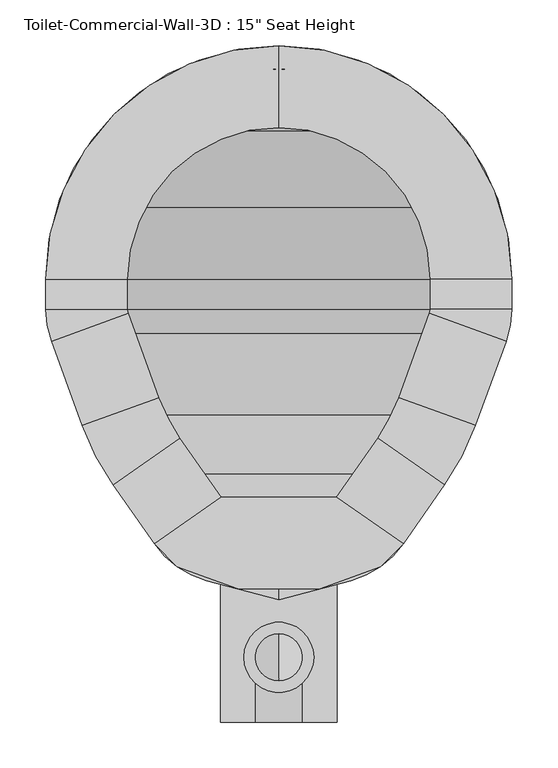
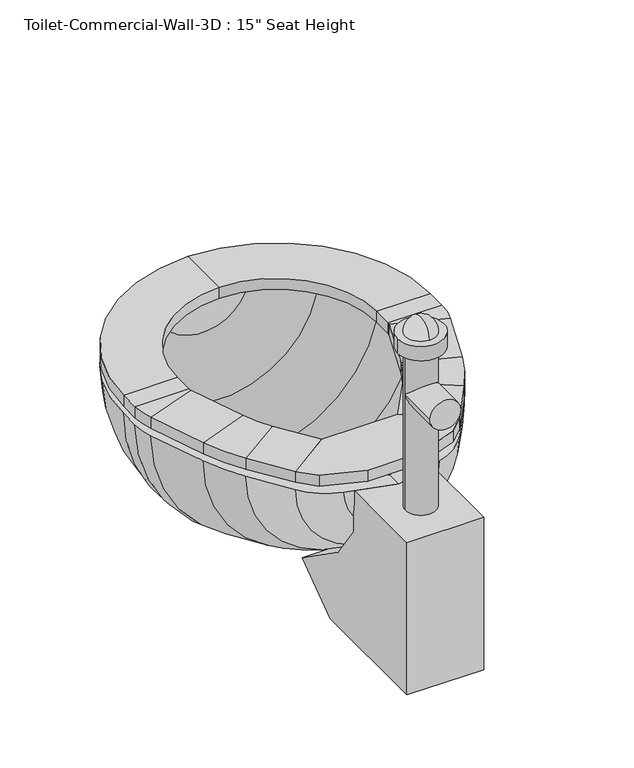
"""IFC4 building model written with IfcOpenShell, lengths in millimetres: flow terminal geometry."""

from ifc_helpers import new_model, si_unit, point, frame, frame_2d, origin, place, context, project, spatial, polyline, circle_curve, ellipse_curve, trimmed, segment, composite_curve, outline, extrude, source, transform, mapped, element, save
from ifc_brep_helpers import plane_surface, cylinder_surface, revolved_surface, advanced_brep


def flow_terminal_fb6ce90a(model_context):
    return source(origin(), model_context, "Body", "SolidModel", [
        extrude(outline(polyline([(467.7541169, 443.4722495), (540.5767337, 392.4813043), (515.6262519, 367.5308226), (449.563909, 343.4860961), (360.2423986, 343.4860961), (294.1800557, 367.5308226), (269.229574, 392.4813043), (342.0521907, 443.4722495), (467.7541169, 443.4722495)])), frame((0.0, 0.0, 355.6), z_axis=(0.0, 0.0, 1.0), x_axis=(1.0, 0.0, 0.0)), (0.0, 0.0, 1.0), 19.05),
        advanced_brep(
        [(467.7541169, 443.4722495, 355.6), (540.5767337, 392.4813043, 355.6), (540.5767337, 392.4813043, 374.65), (467.7541169, 443.4722495, 374.65), (512.8583992, 507.8878403, 355.6), (585.6810159, 456.8968951, 355.6), (585.6810159, 456.8968951, 374.65), (512.8583992, 507.8878403, 374.65), (619.360053, 521.5937234, 355.6), (535.821379, 551.9993141, 355.6), (619.360053, 521.5937234, 374.65), (535.821379, 551.9993141, 374.65), (569.2372501, 643.8086654, 355.6), (652.7759241, 613.4030747, 355.6), (652.7759241, 613.4030747, 374.65), (569.2372501, 643.8086654, 374.65), (658.9031538, 648.1523212, 355.6), (570.0031538, 648.1523212, 355.6), (658.9031538, 648.1523212, 374.65), (570.0031538, 648.1523212, 374.65), (570.0031538, 681.0375, 355.6), (658.9031538, 681.0375, 355.6), (658.9031538, 681.0375, 374.65), (570.0031538, 681.0375, 374.65), (404.9031538, 935.0375, 355.6), (404.9031538, 846.1375, 355.6), (404.9031538, 935.0375, 374.65), (404.9031538, 846.1375, 374.65), (150.9031538, 681.0375, 355.6), (239.8031538, 681.0375, 355.6), (150.9031538, 681.0375, 374.65), (239.8031538, 681.0375, 374.65), (239.8031538, 648.1523212, 355.6), (150.9031538, 648.1523212, 355.6), (150.9031538, 648.1523212, 374.65), (239.8031538, 648.1523212, 374.65), (157.0303835, 613.4030747, 355.6), (240.5690575, 643.8086654, 355.6), (157.0303835, 613.4030747, 374.65), (240.5690575, 643.8086654, 374.65), (273.9849286, 551.9993141, 355.6), (190.4462546, 521.5937234, 355.6), (190.4462546, 521.5937234, 374.65), (273.9849286, 551.9993141, 374.65), (224.1252917, 456.8968951, 355.6), (296.9479084, 507.8878403, 355.6), (224.1252917, 456.8968951, 374.65), (296.9479084, 507.8878403, 374.65), (342.0521907, 443.4722495, 355.6), (342.0521907, 443.4722495, 374.65), (269.229574, 392.4813043, 374.65), (269.229574, 392.4813043, 355.6)],
        [
            (0, 1),
            (1, 2),
            (2, 3),
            (3, 0),
            (0, 4),
            (4, 5),
            (5, 1),
            (5, 6),
            (6, 2),
            (6, 7),
            (7, 3),
            (7, 4),
            (8, 5, circle_curve(frame((356.8099347, 617.1541514, 355.6), z_axis=(0.0, 0.0, -1.0), x_axis=(0.81915204428899, -0.5735764363510486, 0.0)), 279.4)),
            (4, 9, circle_curve(frame((356.8099347, 617.1541514, 355.6), z_axis=(0.0, 0.0, 1.0), x_axis=(0.81915204428899, -0.5735764363510486, 0.0)), 190.5)),
            (9, 8),
            (10, 6, circle_curve(frame((356.8099347, 617.1541514, 374.65), z_axis=(0.0, 0.0, -1.0), x_axis=(0.81915204428899, -0.5735764363510486, 0.0)), 279.4)),
            (8, 10),
            (11, 7, circle_curve(frame((356.8099347, 617.1541514, 374.65), z_axis=(0.0, 0.0, -1.0), x_axis=(0.81915204428899, -0.5735764363510486, 0.0)), 190.5)),
            (10, 11),
            (11, 9),
            (9, 12),
            (12, 13),
            (13, 8),
            (13, 14),
            (14, 10),
            (14, 15),
            (15, 11),
            (15, 12),
            (16, 13, circle_curve(frame((557.3031538, 648.1523212, 355.6), z_axis=(0.0, 0.0, -1.0), x_axis=(0.9396926207859057, -0.3420201433256761, 0.0)), 101.6)),
            (12, 17, circle_curve(frame((557.3031538, 648.1523212, 355.6), z_axis=(0.0, 0.0, 1.0), x_axis=(0.9396926207859057, -0.3420201433256761, 0.0)), 12.7)),
            (17, 16),
            (18, 14, circle_curve(frame((557.3031538, 648.1523212, 374.65), z_axis=(0.0, 0.0, -1.0), x_axis=(0.9396926207859057, -0.3420201433256761, 0.0)), 101.6)),
            (16, 18),
            (19, 15, circle_curve(frame((557.3031538, 648.1523212, 374.65), z_axis=(0.0, 0.0, -1.0), x_axis=(0.9396926207859057, -0.3420201433256761, 0.0)), 12.7)),
            (18, 19),
            (19, 17),
            (17, 20),
            (20, 21),
            (21, 16),
            (21, 22),
            (22, 18),
            (22, 23),
            (23, 19),
            (23, 20),
            (24, 21, circle_curve(frame((404.9031538, 681.0375, 355.6), z_axis=(0.0, 0.0, -1.0), x_axis=(1.0, 0.0, 0.0)), 254.0)),
            (20, 25, circle_curve(frame((404.9031538, 681.0375, 355.6), z_axis=(0.0, 0.0, 1.0), x_axis=(1.0, 0.0, 0.0)), 165.1)),
            (25, 24),
            (26, 22, circle_curve(frame((404.9031538, 681.0375, 374.65), z_axis=(0.0, 0.0, -1.0), x_axis=(1.0, 0.0, 0.0)), 254.0)),
            (24, 26),
            (27, 23, circle_curve(frame((404.9031538, 681.0375, 374.65), z_axis=(0.0, 0.0, -1.0), x_axis=(1.0, 0.0, 0.0)), 165.1)),
            (26, 27),
            (27, 25),
            (28, 24, circle_curve(frame((404.9031538, 681.0375, 355.6), z_axis=(0.0, 0.0, -1.0), x_axis=(0.0, 1.0, 0.0)), 254.0)),
            (25, 29, circle_curve(frame((404.9031538, 681.0375, 355.6), z_axis=(0.0, 0.0, 1.0), x_axis=(0.0, 1.0, 0.0)), 165.1)),
            (29, 28),
            (30, 26, circle_curve(frame((404.9031538, 681.0375, 374.65), z_axis=(0.0, 0.0, -1.0), x_axis=(0.0, 1.0, 0.0)), 254.0)),
            (28, 30),
            (31, 27, circle_curve(frame((404.9031538, 681.0375, 374.65), z_axis=(0.0, 0.0, -1.0), x_axis=(0.0, 1.0, 0.0)), 165.1)),
            (30, 31),
            (31, 29),
            (29, 32),
            (32, 33),
            (33, 28),
            (33, 34),
            (34, 30),
            (34, 35),
            (35, 31),
            (35, 32),
            (36, 33, circle_curve(frame((252.5031538, 648.1523212, 355.6), z_axis=(0.0, 0.0, -1.0), x_axis=(-1.0, 0.0, 0.0)), 101.6)),
            (32, 37, circle_curve(frame((252.5031538, 648.1523212, 355.6), z_axis=(0.0, 0.0, 1.0), x_axis=(-1.0, 0.0, 0.0)), 12.7)),
            (37, 36),
            (38, 34, circle_curve(frame((252.5031538, 648.1523212, 374.65), z_axis=(0.0, 0.0, -1.0), x_axis=(-1.0, 0.0, 0.0)), 101.6)),
            (36, 38),
            (39, 35, circle_curve(frame((252.5031538, 648.1523212, 374.65), z_axis=(0.0, 0.0, -1.0), x_axis=(-1.0, 0.0, 0.0)), 12.7)),
            (38, 39),
            (39, 37),
            (37, 40),
            (40, 41),
            (41, 36),
            (41, 42),
            (42, 38),
            (42, 43),
            (43, 39),
            (43, 40),
            (44, 41, circle_curve(frame((452.9963729, 617.1541514, 355.6), z_axis=(0.0, 0.0, -1.0), x_axis=(-0.939692620785909, -0.3420201433256672, 0.0)), 279.4)),
            (40, 45, circle_curve(frame((452.9963729, 617.1541514, 355.6), z_axis=(0.0, 0.0, 1.0), x_axis=(-0.939692620785909, -0.3420201433256672, 0.0)), 190.5)),
            (45, 44),
            (46, 42, circle_curve(frame((452.9963729, 617.1541514, 374.65), z_axis=(0.0, 0.0, -1.0), x_axis=(-0.939692620785909, -0.3420201433256672, 0.0)), 279.4)),
            (44, 46),
            (47, 43, circle_curve(frame((452.9963729, 617.1541514, 374.65), z_axis=(0.0, 0.0, -1.0), x_axis=(-0.939692620785909, -0.3420201433256672, 0.0)), 190.5)),
            (46, 47),
            (47, 45),
            (48, 49),
            (49, 50),
            (50, 51),
            (51, 48),
            (45, 48),
            (51, 44),
            (50, 46),
            (49, 47),
        ],
        [
            plane_surface(frame((540.5767337, 392.4813043, 437.2995365), z_axis=(-0.5735764363510436, -0.8191520442889937, 0.0), x_axis=(0.8191520442889937, -0.5735764363510436, 0.0))),
            plane_surface(frame((467.7541169, 443.4722495, 355.6), z_axis=(0.0, 0.0, -1.0), x_axis=(0.5735764363510436, 0.8191520442889936, 0.0))),
            plane_surface(frame((540.5767337, 392.4813043, 355.6), z_axis=(0.8191520442889944, -0.5735764363510424, 0.0), x_axis=(0.5735764363510424, 0.8191520442889944, 0.0))),
            plane_surface(frame((540.5767337, 392.4813043, 374.65), z_axis=(0.0, 0.0, 1.0), x_axis=(0.573576436351043, 0.819152044288994, 0.0))),
            plane_surface(frame((467.7541169, 443.4722495, 374.65), z_axis=(-0.819152044288994, 0.573576436351043, 0.0), x_axis=(0.573576436351043, 0.819152044288994, 0.0))),
            plane_surface(frame((356.8099347, 617.1541514, 355.6), z_axis=(0.0, 0.0, -1.0), x_axis=(0.81915204428899, -0.5735764363510486, 0.0))),
            cylinder_surface(frame((356.8099347, 617.1541514, 342.9), z_axis=(0.0, 0.0, 1.0), x_axis=(0.81915204428899, -0.5735764363510486, 0.0)), 279.4),
            plane_surface(frame((356.8099347, 617.1541514, 374.65), z_axis=(0.0, 0.0, 1.0), x_axis=(0.81915204428899, -0.5735764363510486, 0.0))),
            revolved_surface(polyline([(512.8583991370526, 507.8878402751253, 374.65), (512.8583991370526, 507.8878402751253, 355.6)]), (356.8099347, 617.1541514, 342.9), (0.0, 0.0, 1.0)),
            plane_surface(frame((535.821379, 551.9993141, 355.6), z_axis=(0.0, 0.0, -1.0000000000000002), x_axis=(0.3420201433256594, 0.9396926207859119, 0.0))),
            plane_surface(frame((619.360053, 521.5937234, 355.6), z_axis=(0.9396926207859121, -0.3420201433256587, 0.0), x_axis=(0.3420201433256587, 0.9396926207859121, 0.0))),
            plane_surface(frame((619.360053, 521.5937234, 374.65), z_axis=(0.0, 0.0, 1.0), x_axis=(0.34202014332565916, 0.9396926207859119, 0.0))),
            plane_surface(frame((535.821379, 551.9993141, 374.65), z_axis=(-0.9396926207859122, 0.34202014332565833, 0.0), x_axis=(0.34202014332565833, 0.9396926207859122, 0.0))),
            plane_surface(frame((557.3031538, 648.1523212, 355.6), z_axis=(0.0, 0.0, -1.0000000000000002), x_axis=(0.9396926207859058, -0.34202014332567615, 0.0))),
            cylinder_surface(frame((557.3031538, 648.1523212, 342.9), z_axis=(0.0, 0.0, 1.0), x_axis=(0.9396926207859057, -0.3420201433256761, 0.0)), 101.6),
            plane_surface(frame((557.3031538, 648.1523212, 374.65), z_axis=(0.0, 0.0, 1.0000000000000002), x_axis=(0.9396926207859058, -0.34202014332567615, 0.0))),
            revolved_surface(polyline([(569.237250083981, 643.8086653797639, 374.65), (569.237250083981, 643.8086653797639, 355.6)]), (557.3031538, 648.1523212, 342.9), (0.0, 0.0, 1.0)),
            plane_surface(frame((570.0031538, 648.1523212, 355.6), z_axis=(0.0, 0.0, -1.0), x_axis=(0.0, 1.0, 0.0))),
            plane_surface(frame((658.9031538, 648.1523212, 355.6), z_axis=(1.0, 0.0, 0.0), x_axis=(0.0, 1.0, 0.0))),
            plane_surface(frame((658.9031538, 648.1523212, 374.65), z_axis=(0.0, 0.0, 1.0), x_axis=(0.0, 1.0, 0.0))),
            plane_surface(frame((570.0031538, 648.1523212, 374.65), z_axis=(-1.0, 0.0, 0.0), x_axis=(0.0, 1.0, 0.0))),
            plane_surface(frame((404.9031538, 681.0375, 355.6), z_axis=(0.0, 0.0, -1.0), x_axis=(1.0, 0.0, 0.0))),
            cylinder_surface(frame((404.9031538, 681.0375, 342.9), z_axis=(0.0, 0.0, 1.0), x_axis=(1.0, 0.0, 0.0)), 254.0),
            plane_surface(frame((404.9031538, 681.0375, 374.65), z_axis=(0.0, 0.0, 1.0), x_axis=(1.0, 0.0, 0.0))),
            revolved_surface(polyline([(570.0031538, 681.0375, 374.65), (570.0031538, 681.0375, 355.6)]), (404.9031538, 681.0375, 342.9), (0.0, 0.0, 1.0)),
            plane_surface(frame((404.9031538, 681.0375, 355.6), z_axis=(0.0, 0.0, -1.0), x_axis=(0.0, 1.0, 0.0))),
            cylinder_surface(frame((404.9031538, 681.0375, 342.9), z_axis=(0.0, 0.0, 1.0), x_axis=(0.0, 1.0, 0.0)), 254.0),
            plane_surface(frame((404.9031538, 681.0375, 374.65), z_axis=(0.0, 0.0, 1.0), x_axis=(0.0, 1.0, 0.0))),
            revolved_surface(polyline([(404.9031538, 846.1375, 374.65), (404.9031538, 846.1375, 355.6)]), (404.9031538, 681.0375, 342.9), (0.0, 0.0, 1.0)),
            plane_surface(frame((239.8031538, 681.0375, 355.6), z_axis=(0.0, 0.0, -1.0), x_axis=(0.0, -1.0, 0.0))),
            plane_surface(frame((150.9031538, 681.0375, 355.6), z_axis=(-1.0, 0.0, 0.0), x_axis=(0.0, -1.0, 0.0))),
            plane_surface(frame((150.9031538, 681.0375, 374.65), z_axis=(0.0, 0.0, 1.0), x_axis=(0.0, -1.0, 0.0))),
            plane_surface(frame((239.8031538, 681.0375, 374.65), z_axis=(1.0, 0.0, 0.0), x_axis=(0.0, -1.0, 0.0))),
            plane_surface(frame((252.5031538, 648.1523212, 355.6), z_axis=(0.0, 0.0, -1.0), x_axis=(-1.0, 0.0, 0.0))),
            cylinder_surface(frame((252.5031538, 648.1523212, 342.9), z_axis=(0.0, 0.0, 1.0), x_axis=(-1.0, 0.0, 0.0)), 101.6),
            plane_surface(frame((252.5031538, 648.1523212, 374.65), z_axis=(0.0, 0.0, 1.0), x_axis=(-1.0, 0.0, 0.0))),
            revolved_surface(polyline([(239.80315380000002, 648.1523212, 374.65), (239.80315380000002, 648.1523212, 355.6)]), (252.5031538, 648.1523212, 342.9), (0.0, 0.0, 1.0)),
            plane_surface(frame((240.5690575, 643.8086654, 355.6), z_axis=(0.0, 0.0, -1.0), x_axis=(0.3420201433256581, -0.9396926207859123, 0.0))),
            plane_surface(frame((157.0303835, 613.4030747, 355.6), z_axis=(-0.9396926207859122, -0.3420201433256583, 0.0), x_axis=(0.3420201433256583, -0.9396926207859122, 0.0))),
            plane_surface(frame((157.0303835, 613.4030747, 374.65), z_axis=(0.0, 0.0, 1.0), x_axis=(0.34202014332565855, -0.9396926207859121, 0.0))),
            plane_surface(frame((240.5690575, 643.8086654, 374.65), z_axis=(0.9396926207859124, 0.3420201433256579, 0.0), x_axis=(0.3420201433256579, -0.9396926207859124, 0.0))),
            plane_surface(frame((452.9963729, 617.1541514, 355.6), z_axis=(0.0, 0.0, -1.0), x_axis=(-0.939692620785909, -0.3420201433256672, 0.0))),
            cylinder_surface(frame((452.9963729, 617.1541514, 342.9), z_axis=(0.0, 0.0, 1.0), x_axis=(-0.939692620785909, -0.3420201433256672, 0.0)), 279.4),
            plane_surface(frame((452.9963729, 617.1541514, 374.65), z_axis=(0.0, 0.0, 1.0), x_axis=(-0.939692620785909, -0.3420201433256672, 0.0))),
            revolved_surface(polyline([(273.98492864028435, 551.9993140964605, 374.65), (273.98492864028435, 551.9993140964605, 355.6)]), (452.9963729, 617.1541514, 342.9), (0.0, 0.0, 1.0)),
            plane_surface(frame((269.229574, 392.4813043, 248.5004635), z_axis=(0.5735764363510469, -0.8191520442889914, 0.0), x_axis=(0.8191520442889914, 0.5735764363510469, 0.0))),
            plane_surface(frame((296.9479084, 507.8878403, 355.6), z_axis=(0.0, 0.0, -1.0), x_axis=(0.5735764363510465, -0.8191520442889916, 0.0))),
            plane_surface(frame((224.1252917, 456.8968951, 355.6), z_axis=(-0.819152044288991, -0.5735764363510473, 0.0), x_axis=(0.5735764363510473, -0.819152044288991, 0.0))),
            plane_surface(frame((224.1252917, 456.8968951, 374.65), z_axis=(0.0, 0.0, 1.0), x_axis=(0.5735764363510473, -0.819152044288991, 0.0))),
            plane_surface(frame((296.9479084, 507.8878403, 374.65), z_axis=(0.8191520442889914, 0.5735764363510468, 0.0), x_axis=(0.5735764363510468, -0.8191520442889914, 0.0))),
        ],
        [
            (0, [[1, 2, 3, 4]]),
            (1, [[-1, 5, 6, 7]]),
            (2, [[-2, -7, 8, 9]]),
            (3, [[-3, -9, 10, 11]]),
            (4, [[-4, -11, 12, -5]]),
            (5, [[13, -6, 14, 15]]),
            (6, [[16, -8, -13, 17]]),
            (7, [[18, -10, -16, 19]]),
            (8, [[-14, -12, -18, 20]]),
            (9, [[-15, 21, 22, 23]]),
            (10, [[-17, -23, 24, 25]]),
            (11, [[-19, -25, 26, 27]]),
            (12, [[-20, -27, 28, -21]]),
            (13, [[29, -22, 30, 31]]),
            (14, [[32, -24, -29, 33]]),
            (15, [[34, -26, -32, 35]]),
            (16, [[-30, -28, -34, 36]]),
            (17, [[-31, 37, 38, 39]]),
            (18, [[-33, -39, 40, 41]]),
            (19, [[-35, -41, 42, 43]]),
            (20, [[-36, -43, 44, -37]]),
            (21, [[45, -38, 46, 47]]),
            (22, [[48, -40, -45, 49]]),
            (23, [[50, -42, -48, 51]]),
            (24, [[-46, -44, -50, 52]]),
            (25, [[53, -47, 54, 55]]),
            (26, [[56, -49, -53, 57]]),
            (27, [[58, -51, -56, 59]]),
            (28, [[-54, -52, -58, 60]]),
            (29, [[-55, 61, 62, 63]]),
            (30, [[-57, -63, 64, 65]]),
            (31, [[-59, -65, 66, 67]]),
            (32, [[-60, -67, 68, -61]]),
            (33, [[69, -62, 70, 71]]),
            (34, [[72, -64, -69, 73]]),
            (35, [[74, -66, -72, 75]]),
            (36, [[-70, -68, -74, 76]]),
            (37, [[-71, 77, 78, 79]]),
            (38, [[-73, -79, 80, 81]]),
            (39, [[-75, -81, 82, 83]]),
            (40, [[-76, -83, 84, -77]]),
            (41, [[85, -78, 86, 87]]),
            (42, [[88, -80, -85, 89]]),
            (43, [[90, -82, -88, 91]]),
            (44, [[-86, -84, -90, 92]]),
            (45, [[93, 94, 95, 96]]),
            (46, [[-87, 97, -96, 98]]),
            (47, [[-89, -98, -95, 99]]),
            (48, [[-91, -99, -94, 100]]),
            (49, [[-92, -100, -93, -97]]),
        ],
    ),
        advanced_brep(
        [(491.7762702, 919.7194257, 342.9), (404.9031538, 935.0375, 342.9), (404.9031538, 909.6375, 342.9), (483.0889586, 895.8512331, 342.9), (566.547764, 842.6821102, 342.9), (619.7168869, 759.2233048, 342.9), (633.5031538, 681.0375, 342.9), (633.5031538, 648.1523212, 342.9), (628.9077315, 622.0903863, 342.9), (596.6355667, 533.4233422, 342.9), (562.9565296, 468.7265139, 342.9), (525.0728964, 414.6230786, 342.9), (468.1430637, 374.7603806, 342.9), (404.9031538, 357.8152978, 342.9), (404.9031538, 331.5192829, 342.9), (483.6469009, 352.6186063, 342.9), (540.5767337, 392.4813043, 342.9), (585.6810159, 456.8968951, 342.9), (619.360053, 521.5937234, 342.9), (652.7759241, 613.4030747, 342.9), (658.9031538, 648.1523212, 342.9), (658.9031538, 681.0375, 342.9), (643.5850795, 767.9106164, 342.9), (584.5082762, 860.6426224, 342.9), (318.0300374, 919.7194257, 342.9), (225.2980314, 860.6426224, 342.9), (166.2212281, 767.9106164, 342.9), (150.9031538, 681.0375, 342.9), (150.9031538, 648.1523212, 342.9), (157.0303835, 613.4030747, 342.9), (190.4462546, 521.5937234, 342.9), (224.1252917, 456.8968951, 342.9), (269.229574, 392.4813043, 342.9), (326.1594067, 352.6186063, 342.9), (341.663244, 374.7603806, 342.9), (284.7334112, 414.6230786, 342.9), (246.849778, 468.7265139, 342.9), (213.1707409, 533.4233422, 342.9), (180.8985761, 622.0903863, 342.9), (176.3031538, 648.1523212, 342.9), (176.3031538, 681.0375, 342.9), (190.0894207, 759.2233048, 342.9), (243.2585436, 842.6821102, 342.9), (326.7173491, 895.8512331, 342.9)],
        [
            (0, 1, circle_curve(frame((404.9031538, 681.0375, 342.9), z_axis=(0.0, 0.0, 1.0), x_axis=(1.0, 0.0, 0.0)), 254.0)),
            (1, 2),
            (2, 3, circle_curve(frame((404.9031538, 681.0375, 342.9), z_axis=(0.0, 0.0, -1.0), x_axis=(1.0, 0.0, 0.0)), 228.6)),
            (3, 4, circle_curve(frame((404.9031538, 681.0375, 342.9), z_axis=(0.0, 0.0, -1.0), x_axis=(1.0, 0.0, 0.0)), 228.6)),
            (4, 5, circle_curve(frame((404.9031538, 681.0375, 342.9), z_axis=(0.0, 0.0, -1.0), x_axis=(1.0, 0.0, 0.0)), 228.6)),
            (5, 6, circle_curve(frame((404.9031538, 681.0375, 342.9), z_axis=(0.0, 0.0, -1.0), x_axis=(1.0, 0.0, 0.0)), 228.6)),
            (6, 7),
            (7, 8, circle_curve(frame((557.3031538, 648.1523212, 342.9), z_axis=(0.0, 0.0, -1.0), x_axis=(1.0, 0.0, 0.0)), 76.2)),
            (8, 9),
            (9, 10, circle_curve(frame((334.0854485, 628.9837703, 342.9), z_axis=(0.0, 0.0, -1.0), x_axis=(1.0, 0.0, 0.0)), 279.4)),
            (10, 11),
            (11, 12, circle_curve(frame((441.8470487, 472.8984446, 342.9), z_axis=(0.0, 0.0, -1.0), x_axis=(1.0, 0.0, 0.0)), 101.6)),
            (12, 13),
            (13, 14),
            (14, 15),
            (15, 16, circle_curve(frame((457.350886, 450.7566703, 342.9), z_axis=(0.0, 0.0, 1.0), x_axis=(1.0, 0.0, 0.0)), 101.6)),
            (16, 17),
            (17, 18, circle_curve(frame((356.8099347, 617.1541514, 342.9), z_axis=(0.0, 0.0, 1.0), x_axis=(1.0, 0.0, 0.0)), 279.4)),
            (18, 19),
            (19, 20, circle_curve(frame((557.3031538, 648.1523212, 342.9), z_axis=(0.0, 0.0, 1.0), x_axis=(1.0, 0.0, 0.0)), 101.6)),
            (20, 21),
            (21, 22, circle_curve(frame((404.9031538, 681.0375, 342.9), z_axis=(0.0, 0.0, 1.0), x_axis=(1.0, 0.0, 0.0)), 254.0)),
            (22, 23, circle_curve(frame((404.9031538, 681.0375, 342.9), z_axis=(0.0, 0.0, 1.0), x_axis=(1.0, 0.0, 0.0)), 254.0)),
            (23, 0, circle_curve(frame((404.9031538, 681.0375, 342.9), z_axis=(0.0, 0.0, 1.0), x_axis=(1.0, 0.0, 0.0)), 254.0)),
            (24, 25, circle_curve(frame((404.9031538, 681.0375, 342.9), z_axis=(0.0, 0.0, 1.0), x_axis=(-1.0, 0.0, 0.0)), 254.0)),
            (25, 26, circle_curve(frame((404.9031538, 681.0375, 342.9), z_axis=(0.0, 0.0, 1.0), x_axis=(-1.0, 0.0, 0.0)), 254.0)),
            (26, 27, circle_curve(frame((404.9031538, 681.0375, 342.9), z_axis=(0.0, 0.0, 1.0), x_axis=(-1.0, 0.0, 0.0)), 254.0)),
            (27, 28),
            (28, 29, circle_curve(frame((252.5031538, 648.1523212, 342.9), z_axis=(0.0, 0.0, 1.0), x_axis=(-1.0, 0.0, 0.0)), 101.6)),
            (29, 30),
            (30, 31, circle_curve(frame((452.9963729, 617.1541514, 342.9), z_axis=(0.0, 0.0, 1.0), x_axis=(-1.0, 0.0, 0.0)), 279.4)),
            (31, 32),
            (32, 33, circle_curve(frame((352.4554217, 450.7566703, 342.9), z_axis=(0.0, 0.0, 1.0), x_axis=(-1.0, 0.0, 0.0)), 101.6)),
            (33, 14),
            (13, 34),
            (34, 35, circle_curve(frame((367.9592589, 472.8984446, 342.9), z_axis=(0.0, 0.0, -1.0), x_axis=(-1.0, 0.0, 0.0)), 101.6)),
            (35, 36),
            (36, 37, circle_curve(frame((475.7208592, 628.9837703, 342.9), z_axis=(0.0, 0.0, -1.0), x_axis=(-1.0, 0.0, 0.0)), 279.4)),
            (37, 38),
            (38, 39, circle_curve(frame((252.5031538, 648.1523212, 342.9), z_axis=(0.0, 0.0, -1.0), x_axis=(-1.0, 0.0, 0.0)), 76.2)),
            (39, 40),
            (40, 41, circle_curve(frame((404.9031538, 681.0375, 342.9), z_axis=(0.0, 0.0, -1.0), x_axis=(-1.0, 0.0, 0.0)), 228.6)),
            (41, 42, circle_curve(frame((404.9031538, 681.0375, 342.9), z_axis=(0.0, 0.0, -1.0), x_axis=(-1.0, 0.0, 0.0)), 228.6)),
            (42, 43, circle_curve(frame((404.9031538, 681.0375, 342.9), z_axis=(0.0, 0.0, -1.0), x_axis=(-1.0, 0.0, 0.0)), 228.6)),
            (43, 2, circle_curve(frame((404.9031538, 681.0375, 342.9), z_axis=(0.0, 0.0, -1.0), x_axis=(-1.0, 0.0, 0.0)), 228.6)),
            (1, 24, circle_curve(frame((404.9031538, 681.0375, 342.9), z_axis=(0.0, 0.0, 1.0), x_axis=(-1.0, 0.0, 0.0)), 254.0)),
            (0, 24, circle_curve(frame((404.9031538, 919.7194257, 342.9), z_axis=(0.0, 1.0, 0.0), x_axis=(1.0, 0.0, 0.0)), 86.8731164)),
            (43, 3, circle_curve(frame((404.9031538, 895.8512331, 342.9), z_axis=(0.0, -1.0, 0.0), x_axis=(1.0, 0.0, 0.0)), 78.1858048)),
            (42, 4, circle_curve(frame((404.9031538, 842.6821102, 342.9), z_axis=(0.0, -1.0, 0.0), x_axis=(1.0, 0.0, 0.0)), 161.6446102)),
            (41, 5, circle_curve(frame((404.9031538, 759.2233048, 342.9), z_axis=(0.0, -1.0, 0.0), x_axis=(1.0, 0.0, 0.0)), 214.8137331)),
            (40, 6, circle_curve(frame((404.9031538, 681.0375, 342.9), z_axis=(0.0, -1.0, 0.0), x_axis=(1.0, 0.0, 0.0)), 228.6)),
            (39, 7, circle_curve(frame((404.9031538, 648.1523212, 342.9), z_axis=(0.0, -1.0, 0.0), x_axis=(1.0, 0.0, 0.0)), 228.6)),
            (38, 8, circle_curve(frame((404.9031538, 622.0903863, 342.9), z_axis=(0.0, -1.0, 0.0), x_axis=(1.0, 0.0, 0.0)), 224.0045777)),
            (37, 9, circle_curve(frame((404.9031538, 533.4233422, 342.9), z_axis=(0.0, -1.0, 0.0), x_axis=(1.0, 0.0, 0.0)), 191.7324129)),
            (36, 10, circle_curve(frame((404.9031538, 468.7265139, 342.9), z_axis=(0.0, -1.0, 0.0), x_axis=(1.0, 0.0, 0.0)), 158.0533758)),
            (35, 11, circle_curve(frame((404.9031538, 414.6230786, 342.9), z_axis=(0.0, -1.0, 0.0), x_axis=(1.0, 0.0, 0.0)), 120.1697426)),
            (34, 12, circle_curve(frame((404.9031538, 374.7603806, 342.9), z_axis=(0.0, -1.0, 0.0), x_axis=(1.0, 0.0, 0.0)), 63.2399099)),
            (33, 15, circle_curve(frame((404.9031538, 352.6186063, 342.9), z_axis=(0.0, -1.0, 0.0), x_axis=(1.0, 0.0, 0.0)), 78.7437471)),
            (32, 16, circle_curve(frame((404.9031538, 392.4813043, 342.9), z_axis=(0.0, -1.0, 0.0), x_axis=(1.0, 0.0, 0.0)), 135.6735798)),
            (31, 17, circle_curve(frame((404.9031538, 456.8968951, 342.9), z_axis=(0.0, -1.0, 0.0), x_axis=(1.0, 0.0, 0.0)), 180.7778621)),
            (30, 18, circle_curve(frame((404.9031538, 521.5937234, 342.9), z_axis=(0.0, -1.0, 0.0), x_axis=(1.0, 0.0, 0.0)), 214.4568992)),
            (29, 19, circle_curve(frame((404.9031538, 613.4030747, 342.9), z_axis=(0.0, -1.0, 0.0), x_axis=(1.0, 0.0, 0.0)), 247.8727703)),
            (28, 20, circle_curve(frame((404.9031538, 648.1523212, 342.9), z_axis=(0.0, -1.0, 0.0), x_axis=(1.0, 0.0, 0.0)), 254.0)),
            (27, 21, circle_curve(frame((404.9031538, 681.0375, 342.9), z_axis=(0.0, -1.0, 0.0), x_axis=(1.0, 0.0, 0.0)), 254.0)),
            (26, 22, circle_curve(frame((404.9031538, 767.9106164, 342.9), z_axis=(0.0, -1.0, 0.0), x_axis=(1.0, 0.0, 0.0)), 238.6819257)),
            (25, 23, circle_curve(frame((404.9031538, 860.6426224, 342.9), z_axis=(0.0, -1.0, 0.0), x_axis=(1.0, 0.0, 0.0)), 179.6051224)),
        ],
        [
            plane_surface(frame((404.9031538, 1040.2477448, 342.9), z_axis=(0.0, 0.0, 1.0), x_axis=(1.0, 0.0, 0.0))),
            plane_surface(frame((404.9031538, 1040.2477448, 342.9), z_axis=(0.0, 0.0, 1.0), x_axis=(-1.0, 0.0, 0.0))),
            revolved_surface(trimmed(ellipse_curve(frame((404.9031538, 681.0375, 342.9), z_axis=(0.0, 0.0, 1.0), x_axis=(1.0, 0.0, 0.0)), 254.0, 254.0), [point((491.7762702, 919.7194257, 342.9))], [point((404.9031538, 935.0375, 342.9))], True, "CARTESIAN"), (404.9031538, 1040.2477448, 342.9), (0.0, 1.0, 0.0)),
            revolved_surface(trimmed(ellipse_curve(frame((404.9031538, 681.0375, 342.9), z_axis=(0.0, 0.0, -1.0), x_axis=(1.0, 0.0, 0.0)), 228.6, 228.6), [point((404.9031538, 909.6375, 342.9))], [point((483.0889586, 895.8512331, 342.9))], True, "CARTESIAN"), (404.9031538, 1040.2477448, 342.9), (0.0, 1.0, 0.0)),
            revolved_surface(trimmed(ellipse_curve(frame((404.9031538, 681.0375, 342.9), z_axis=(0.0, 0.0, -1.0), x_axis=(1.0, 0.0, 0.0)), 228.6, 228.6), [point((483.0889586, 895.8512331, 342.9))], [point((566.547764, 842.6821102, 342.9))], True, "CARTESIAN"), (404.9031538, 1040.2477448, 342.9), (0.0, 1.0, 0.0)),
            revolved_surface(trimmed(ellipse_curve(frame((404.9031538, 681.0375, 342.9), z_axis=(0.0, 0.0, -1.0), x_axis=(1.0, 0.0, 0.0)), 228.6, 228.6), [point((566.547764, 842.6821102, 342.9))], [point((619.7168869, 759.2233048, 342.9))], True, "CARTESIAN"), (404.9031538, 1040.2477448, 342.9), (0.0, 1.0, 0.0)),
            revolved_surface(trimmed(ellipse_curve(frame((404.9031538, 681.0375, 342.9), z_axis=(0.0, 0.0, -1.0), x_axis=(1.0, 0.0, 0.0)), 228.6, 228.6), [point((619.7168869, 759.2233048, 342.9))], [point((633.5031538, 681.0375, 342.9))], True, "CARTESIAN"), (404.9031538, 1040.2477448, 342.9), (0.0, 1.0, 0.0)),
            revolved_surface(polyline([(633.5031538, 681.0375, 342.9), (633.5031538, 648.1523212, 342.9)]), (404.9031538, 1040.2477448, 342.9), (0.0, 1.0, 0.0)),
            revolved_surface(trimmed(ellipse_curve(frame((557.3031538, 648.1523212, 342.9), z_axis=(0.0, 0.0, -1.0), x_axis=(1.0, 0.0, 0.0)), 76.2, 76.2), [point((633.5031538, 648.1523212, 342.9))], [point((628.9077315, 622.0903863, 342.9))], True, "CARTESIAN"), (404.9031538, 1040.2477448, 342.9), (0.0, 1.0, 0.0)),
            revolved_surface(polyline([(628.9077315, 622.0903863, 342.9), (596.6355667, 533.4233422, 342.9)]), (404.9031538, 1040.2477448, 342.9), (0.0, 1.0, 0.0)),
            revolved_surface(trimmed(ellipse_curve(frame((334.0854485, 628.9837703, 342.9), z_axis=(0.0, 0.0, -1.0), x_axis=(1.0, 0.0, 0.0)), 279.4, 279.4), [point((596.6355667, 533.4233422, 342.9))], [point((562.9565296, 468.7265139, 342.9))], True, "CARTESIAN"), (404.9031538, 1040.2477448, 342.9), (0.0, 1.0, 0.0)),
            revolved_surface(polyline([(562.9565296, 468.7265139, 342.9), (525.0728964, 414.6230786, 342.9)]), (404.9031538, 1040.2477448, 342.9), (0.0, 1.0, 0.0)),
            revolved_surface(trimmed(ellipse_curve(frame((441.8470487, 472.8984446, 342.9), z_axis=(0.0, 0.0, -1.0), x_axis=(1.0, 0.0, 0.0)), 101.6, 101.6), [point((525.0728964, 414.6230786, 342.9))], [point((468.1430637, 374.7603806, 342.9))], True, "CARTESIAN"), (404.9031538, 1040.2477448, 342.9), (0.0, 1.0, 0.0)),
            revolved_surface(polyline([(468.1430637, 374.7603806, 342.9), (404.9031538, 357.8152978, 342.9)]), (404.9031538, 1040.2477448, 342.9), (0.0, 1.0, 0.0)),
            revolved_surface(polyline([(404.9031538, 331.5192829, 342.9), (483.6469009, 352.6186063, 342.9)]), (404.9031538, 1040.2477448, 342.9), (0.0, 1.0, 0.0)),
            revolved_surface(trimmed(ellipse_curve(frame((457.350886, 450.7566703, 342.9), z_axis=(0.0, 0.0, 1.0), x_axis=(1.0, 0.0, 0.0)), 101.6, 101.6), [point((483.6469009, 352.6186063, 342.9))], [point((540.5767337, 392.4813043, 342.9))], True, "CARTESIAN"), (404.9031538, 1040.2477448, 342.9), (0.0, 1.0, 0.0)),
            revolved_surface(polyline([(540.5767337, 392.4813043, 342.9), (585.6810159, 456.8968951, 342.9)]), (404.9031538, 1040.2477448, 342.9), (0.0, 1.0, 0.0)),
            revolved_surface(trimmed(ellipse_curve(frame((356.8099347, 617.1541514, 342.9), z_axis=(0.0, 0.0, 1.0), x_axis=(1.0, 0.0, 0.0)), 279.4, 279.4), [point((585.6810159, 456.8968951, 342.9))], [point((619.360053, 521.5937234, 342.9))], True, "CARTESIAN"), (404.9031538, 1040.2477448, 342.9), (0.0, 1.0, 0.0)),
            revolved_surface(polyline([(619.360053, 521.5937234, 342.9), (652.7759241, 613.4030747, 342.9)]), (404.9031538, 1040.2477448, 342.9), (0.0, 1.0, 0.0)),
            revolved_surface(trimmed(ellipse_curve(frame((557.3031538, 648.1523212, 342.9), z_axis=(0.0, 0.0, 1.0), x_axis=(1.0, 0.0, 0.0)), 101.6, 101.6), [point((652.7759241, 613.4030747, 342.9))], [point((658.9031538, 648.1523212, 342.9))], True, "CARTESIAN"), (404.9031538, 1040.2477448, 342.9), (0.0, 1.0, 0.0)),
            cylinder_surface(frame((404.9031538, 1040.2477448, 342.9), z_axis=(0.0, 1.0, 0.0), x_axis=(1.0, 0.0, 0.0)), 254.0),
            revolved_surface(trimmed(ellipse_curve(frame((404.9031538, 681.0375, 342.9), z_axis=(0.0, 0.0, 1.0), x_axis=(1.0, 0.0, 0.0)), 254.0, 254.0), [point((658.9031538, 681.0375, 342.9))], [point((643.5850795, 767.9106164, 342.9))], True, "CARTESIAN"), (404.9031538, 1040.2477448, 342.9), (0.0, 1.0, 0.0)),
            revolved_surface(trimmed(ellipse_curve(frame((404.9031538, 681.0375, 342.9), z_axis=(0.0, 0.0, 1.0), x_axis=(1.0, 0.0, 0.0)), 254.0, 254.0), [point((643.5850795, 767.9106164, 342.9))], [point((584.5082762, 860.6426224, 342.9))], True, "CARTESIAN"), (404.9031538, 1040.2477448, 342.9), (0.0, 1.0, 0.0)),
            revolved_surface(trimmed(ellipse_curve(frame((404.9031538, 681.0375, 342.9), z_axis=(0.0, 0.0, 1.0), x_axis=(1.0, 0.0, 0.0)), 254.0, 254.0), [point((584.5082762, 860.6426224, 342.9))], [point((491.7762702, 919.7194257, 342.9))], True, "CARTESIAN"), (404.9031538, 1040.2477448, 342.9), (0.0, 1.0, 0.0)),
        ],
        [
            (0, [[1, 2, 3, 4, 5, 6, 7, 8, 9, 10, 11, 12, 13, 14, 15, 16, 17, 18, 19, 20, 21, 22, 23, 24]]),
            (1, [[25, 26, 27, 28, 29, 30, 31, 32, 33, 34, -14, 35, 36, 37, 38, 39, 40, 41, 42, 43, 44, 45, -2, 46]]),
            (2, [[-1, 47, -46]]),
            (3, [[48, -3, -45]]),
            (4, [[49, -4, -48, -44]]),
            (5, [[50, -5, -49, -43]]),
            (6, [[51, -6, -50, -42]]),
            (7, [[52, -7, -51, -41]]),
            (8, [[53, -8, -52, -40]]),
            (9, [[54, -9, -53, -39]]),
            (10, [[55, -10, -54, -38]]),
            (11, [[56, -11, -55, -37]]),
            (12, [[57, -12, -56, -36]]),
            (13, [[-13, -57, -35]]),
            (14, [[58, -15, -34]]),
            (15, [[59, -16, -58, -33]]),
            (16, [[60, -17, -59, -32]]),
            (17, [[61, -18, -60, -31]]),
            (18, [[62, -19, -61, -30]]),
            (19, [[63, -20, -62, -29]]),
            (20, [[64, -21, -63, -28]]),
            (21, [[65, -22, -64, -27]]),
            (22, [[66, -23, -65, -26]]),
            (23, [[-47, -24, -66, -25]]),
        ],
    ),
        advanced_brep(
        [(404.9031538, 243.3551912, 647.7), (404.9031538, 294.5903563, 647.7), (404.9031538, 268.9727737, 673.3175826), (404.9031538, 268.9727737, 647.7)],
        [
            (0, 1, circle_curve(frame((404.9031538, 268.9727737, 647.7), z_axis=(0.0, 0.0, 1.0), x_axis=(0.0, 1.0, 0.0)), 25.6175826)),
            (1, 2, circle_curve(frame((404.9031538, 268.9727737, 647.7), z_axis=(1.0, 0.0, 0.0), x_axis=(0.0, -1.0, 0.0)), 25.6175826)),
            (2, 0, circle_curve(frame((404.9031538, 268.9727737, 647.7), z_axis=(1.0, 0.0, 0.0), x_axis=(0.0, 1.0, 0.0)), 25.6175826)),
            (1, 0, circle_curve(frame((404.9031538, 268.9727737, 647.7), z_axis=(0.0, 0.0, 1.0), x_axis=(0.0, 1.0, 0.0)), 25.6175826)),
            (3, 1),
            (0, 3),
        ],
        [
            revolved_surface(trimmed(ellipse_curve(frame((404.9031538, 268.9727737, 647.7), z_axis=(-1.0, 0.0, 0.0), x_axis=(0.0, -1.0, 0.0)), 25.6175826, 25.6175826), [point((404.9031538, 268.9727737, 673.3175826))], [point((404.9031538, 294.5903563, 647.7))], True, "CARTESIAN"), (404.9031538, 268.9727737, 712.3277273), (0.0, 0.0, -1.0)),
            plane_surface(frame((404.9031538, 268.9727737, 647.7), z_axis=(0.0, 0.0, -1.0), x_axis=(0.0, 1.0, 0.0))),
        ],
        [
            (0, [[1, 2, 3]]),
            (0, [[4, -3, -2]]),
            (1, [[5, -1, 6]]),
            (1, [[-6, -4, -5]]),
        ],
    ),
        extrude(outline(composite_curve([segment(trimmed(circle_curve(frame_2d((404.9031538, 268.9727737)), 38.1), [point((366.8031538, 268.9727737))], [point((443.0031538, 268.9727737))], False, "CARTESIAN"), True, "CONTINUOUS"), segment(trimmed(circle_curve(frame_2d((404.9031538, 268.9727737)), 38.1), [point((443.0031538, 268.9727737))], [point((366.8031538, 268.9727737))], False, "CARTESIAN"), True, "CONTINUOUS")], self_intersect=False)), frame((0.0, 0.0, 622.3), z_axis=(0.0, 0.0, 1.0), x_axis=(1.0, 0.0, 0.0)), (0.0, 0.0, 1.0), 25.4),
        extrude(outline(composite_curve([segment(trimmed(circle_curve(frame_2d((544.2113641, 404.9031538)), 25.4), [point((544.2113641, 379.5031538))], [point((544.2113641, 430.3031538))], False, "CARTESIAN"), True, "CONTINUOUS"), segment(trimmed(circle_curve(frame_2d((544.2113641, 404.9031538)), 25.4), [point((544.2113641, 430.3031538))], [point((544.2113641, 379.5031538))], False, "CARTESIAN"), True, "CONTINUOUS")], self_intersect=False)), frame((0.0, 198.4375, 0.0), z_axis=(0.0, 1.0, 0.0), x_axis=(0.0, 0.0, 1.0)), (0.0, 0.0, 1.0), 70.64375),
        extrude(outline(polyline([(351.2412941, 342.9), (351.2412941, 269.296452), (394.9478185, 206.8770663), (498.9801282, 134.0328588), (418.4829017, 76.2), (198.4375, 76.2), (198.4375, 342.9), (351.2412941, 342.9)])), frame((341.4031538, 0.0, 0.0), z_axis=(1.0, 0.0, 0.0), x_axis=(0.0, 1.0, 0.0)), (0.0, 0.0, 1.0), 127.0),
        extrude(outline(composite_curve([segment(trimmed(circle_curve(frame_2d((404.9031538, 268.9727737)), 25.4), [point((379.5031538, 268.9727737))], [point((430.3031538, 268.9727737))], False, "CARTESIAN"), True, "CONTINUOUS"), segment(trimmed(circle_curve(frame_2d((404.9031538, 268.9727737)), 25.4), [point((430.3031538, 268.9727737))], [point((379.5031538, 268.9727737))], False, "CARTESIAN"), True, "CONTINUOUS")], self_intersect=False)), frame((0.0, 0.0, 342.9), z_axis=(0.0, 0.0, 1.0), x_axis=(1.0, 0.0, 0.0)), (0.0, 0.0, 1.0), 279.4),
    ])


if __name__ == "__main__":
    model = new_model("IFC4")
    model_context = context("Model", 3, world=origin())
    ifc_project = project(units=[si_unit("LENGTHUNIT", "METRE", prefix="MILLI")], contexts=[model_context])
    site = spatial("IfcSite", under=ifc_project)
    building = spatial("IfcBuilding", under=site)
    placement = place(None, origin())
    flow_terminal_shape = flow_terminal_fb6ce90a(model_context)
    element("IfcFlowTerminal", 1, ObjectType="Toilet-Commercial-Wall-3D : 15\" Seat Height", at=placement, inside=building, context=model_context, shape_type="MappedRepresentation", body=[
        mapped(flow_terminal_shape, transform((0.0, 0.0, 0.0), x_axis=(1.0, 0.0, 0.0), y_axis=(0.0, 1.0, 0.0), z_axis=(0.0, 0.0, 1.0))),
    ])
    save(model, "model.ifc")

# Revit data of these elements
# Type "Toilet-Commercial-Wall-3D : 15\" Seat Height"
#   Assembly Code = "D2010110"
#   Mounting Height = 1' - 3"
#   Piping Material = Metal - Steel, Polished
#   Toilet - Bowl Material = Porcelain - Ivory
#   Toilet - Seat Material = Laminate - Ivory,Matte
#   Default Elevation = 0
# Element 1 (IfcFlowTerminal, "Toilet-Commercial-Wall-3D : 15\" Seat Height")
#   Materials on its faces: "Laminate - Ivory,Matte", "Porcelain - Ivory", "Metal - Steel, Polished"
# Materials
#   "Metal - Steel, Polished": class "Unassigned", colour RGB 57 57 57, transparency 0
#   "Porcelain - Ivory": class "Unassigned", colour RGB 247 247 239, transparency 0
#   "Laminate - Ivory,Matte": class "Unassigned", colour RGB 247 247 239, transparency 0, Description = "Laminate"
